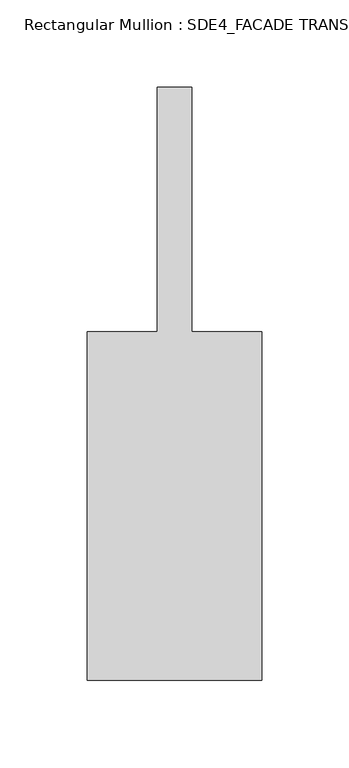
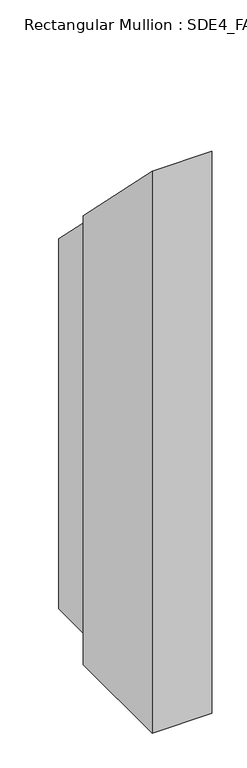
"""IFC4 building model written with IfcOpenShell, lengths in millimetres: member geometry, Rectangular Mullion : SDE4_FACADE TRANSOM TYPE 1."""

from ifc_helpers import new_model, si_unit, origin, place, context, project, spatial, faceted_brep, source, transform, mapped, element, save


def rectangular_mullion_sde4_facade_transom_type_1_69795633(model_context):
    return source(origin(), model_context, "Body", "Brep", [
        faceted_brep([(50.0, -132.5, -861.5375289), (-50.0, -132.5, -861.5375289), (-50.0, 67.5, -861.5375289), (-10.0, 67.5, -861.5375289), (-10.0, 207.5, -861.5375289), (10.0, 207.5, -861.5375289), (10.0, 67.5, -861.5375289), (50.0, 67.5, -861.5375289), (50.0, 67.5, -67.5), (50.0, -132.5, 132.5), (10.0, 67.5, -67.5), (10.0, 207.5, -207.5), (-10.0, 207.5, -207.5), (-10.0, 67.5, -67.5), (-50.0, 67.5, -67.5), (-50.0, -132.5, 132.5)], [[[0, 1, 2, 3, 4, 5, 6, 7]], [[8, 9, 0, 7]], [[10, 8, 7, 6]], [[11, 10, 6, 5]], [[12, 11, 5, 4]], [[13, 12, 4, 3]], [[14, 13, 3, 2]], [[15, 14, 2, 1]], [[9, 15, 1, 0]], [[9, 8, 10, 11, 12, 13, 14, 15]]]),
    ])


if __name__ == "__main__":
    model = new_model("IFC4")
    model_context = context("Model", 3, world=origin())
    ifc_project = project(units=[si_unit("LENGTHUNIT", "METRE", prefix="MILLI")], contexts=[model_context])
    site = spatial("IfcSite", under=ifc_project)
    building = spatial("IfcBuilding", under=site)
    placement = place(None, origin())
    rectangular_mullion_sde4_facade_transom_type_1_shape = rectangular_mullion_sde4_facade_transom_type_1_69795633(model_context)
    element("IfcMember", 1, ObjectType="Rectangular Mullion : SDE4_FACADE TRANSOM TYPE 1", at=placement, inside=building, context=model_context, shape_type="MappedRepresentation", body=[
        mapped(rectangular_mullion_sde4_facade_transom_type_1_shape, transform((0.0, 0.0, 0.0), x_axis=(1.0, 0.0, 0.0), y_axis=(0.0, 1.0, 0.0), z_axis=(0.0, 0.0, 1.0))),
    ])
    save(model, "model.ifc")

# Revit data of these elements
# Type "Rectangular Mullion : SDE4_FACADE TRANSOM TYPE 1"
#   built-in parameter 1007322 = 1.11549 (stored number, unit not read)
#   built-in parameter 1007321 = 0.164042 (stored number, unit not read)
#   built-in parameter 1007320 = 0.164042 (stored number, unit not read)
